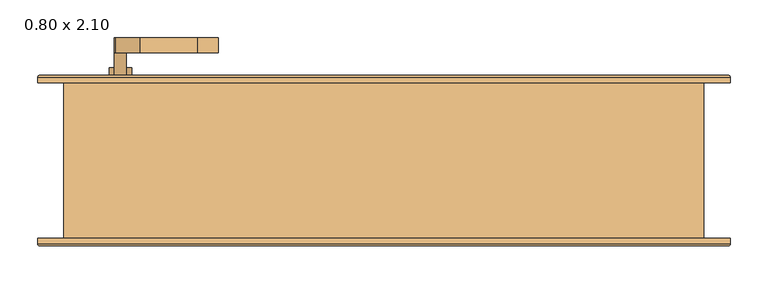
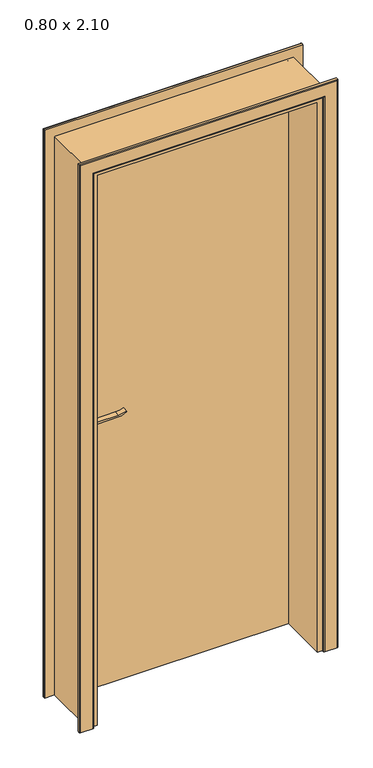
"""IFC4 building model written with IfcOpenShell, lengths in millimetres: door geometry, .CC_ND 300_PORTA SIMPLES DE ABRIR_COM EXTENSÃO : 0.80 x 2.10."""

import ifcopenshell
import ifcopenshell.guid

model = None  # the IFC model being written
_history = None  # IfcOwnerHistory: only IFC2X3 demands one
_inside = {}  # id of a spatial element -> (the spatial element, [elements in it])
_under = {}  # id of a project, library or spatial element -> (it, [spatial elements below it])
_declared = {}  # id of a project -> (the project, [libraries it declares])
_typed = {}  # id of a type object -> (the type object, [elements of that type])
_made_of = {}  # id of a material, layer set ... -> (it, [elements and type objects made of it])


def new_model(schema):
    """Start an empty IFC model of exactly this schema.

    Asked for "IFC4X3", IfcOpenShell would pick the latest addendum, in which some entities
    have other attributes; the version numbers below select the first issue.
    IFC2X3 requires an IfcOwnerHistory on every rooted entity: one is made here for all.
    """
    global model, _history
    if schema == "IFC4X3":
        model = ifcopenshell.file(schema_version=(4, 3, 0, 0))
    else:
        model = ifcopenshell.file(schema=schema)
    _inside.clear()
    _under.clear()
    _declared.clear()
    _typed.clear()
    _made_of.clear()
    _history = None
    if model.schema == "IFC2X3":
        org = make("IfcOrganization", Name="unknown")
        user = make(
            "IfcPersonAndOrganization",
            ThePerson=make("IfcPerson", FamilyName="unknown"),
            TheOrganization=org,
        )
        app = make(
            "IfcApplication",
            ApplicationDeveloper=org,
            Version="unknown",
            ApplicationFullName="unknown",
            ApplicationIdentifier="unknown",
        )
        _history = make(
            "IfcOwnerHistory",
            OwningUser=user,
            OwningApplication=app,
            ChangeAction="ADDED",
            CreationDate=0,
        )
    return model


def make(cls, **values):
    """One entity of the class cls with the attributes given. An attribute that is None is left unset."""
    return model.create_entity(
        cls, **{name: value for name, value in values.items() if value is not None}
    )


def rooted(cls, **values):
    """An entity with a GlobalId (a new one), such as an element, a storey or a relation."""
    return make(cls, GlobalId=ifcopenshell.guid.new(), OwnerHistory=_history, **values)


def si_unit(unit_type, name, prefix=None):
    """IfcSIUnit, for example si_unit("LENGTHUNIT", "METRE", prefix="MILLI")."""
    return make("IfcSIUnit", UnitType=unit_type, Prefix=prefix, Name=name)


def assignment(units):
    """IfcUnitAssignment: the units of a project."""
    return None if units is None else make("IfcUnitAssignment", Units=units)


def point(xyz):
    """IfcCartesianPoint."""
    return None if xyz is None else make("IfcCartesianPoint", Coordinates=xyz)


def direction(xyz):
    """IfcDirection."""
    return None if xyz is None else make("IfcDirection", DirectionRatios=xyz)


def frame(location, z_axis=None, x_axis=None):
    """IfcAxis2Placement3D, a coordinate frame: its origin and axes. An axis left out is left unset."""
    return make(
        "IfcAxis2Placement3D",
        Location=point(location),
        Axis=direction(z_axis),
        RefDirection=direction(x_axis),
    )


def frame_2d(location, x_axis=None):
    """IfcAxis2Placement2D, a coordinate frame in the plane: its origin and x axis."""
    return make(
        "IfcAxis2Placement2D", Location=point(location), RefDirection=direction(x_axis)
    )


def origin():
    """The frame at (0, 0, 0) with its axes left unset."""
    return frame((0.0, 0.0, 0.0))


def origin_with_axes():
    """The frame at (0, 0, 0) with the z axis (0, 0, 1) and the x axis (1, 0, 0) written out."""
    return frame((0.0, 0.0, 0.0), z_axis=(0.0, 0.0, 1.0), x_axis=(1.0, 0.0, 0.0))


def place(relative_to, where):
    """IfcLocalPlacement: puts the frame where relative to a parent placement (None: the world)."""
    return make(
        "IfcLocalPlacement", PlacementRelTo=relative_to, RelativePlacement=where
    )


def context(
    kind, dimensions, precision=None, world=None, true_north=None, identifier=None
):
    """IfcGeometricRepresentationContext, for example the 3D "Model" context."""
    return make(
        "IfcGeometricRepresentationContext",
        ContextIdentifier=identifier,
        ContextType=kind,
        CoordinateSpaceDimension=dimensions,
        Precision=precision,
        WorldCoordinateSystem=world,
        TrueNorth=true_north,
    )


def project(units=None, contexts=None):
    """IfcProject with its units and contexts."""
    return rooted(
        "IfcProject",
        Name="project",
        RepresentationContexts=contexts,
        UnitsInContext=assignment(units),
    )


def spatial(cls, under=None, at=None, **own):
    """A site, building, storey or space (cls), placed at a placement, below another one or the project."""
    s = rooted(cls, ObjectPlacement=at, **own)
    if under is not None:
        _under.setdefault(under.id(), (under, []))[1].append(s)
    return s


def polyline(points):
    """IfcPolyline through the points."""
    return make("IfcPolyline", Points=[point(p) for p in points])


def circle_curve(where, radius):
    """IfcCircle in the frame where."""
    return make("IfcCircle", Position=where, Radius=radius)


def ellipse_curve(where, semi_axis1, semi_axis2):
    """IfcEllipse in the frame where."""
    return make(
        "IfcEllipse", Position=where, SemiAxis1=semi_axis1, SemiAxis2=semi_axis2
    )


def trimmed(basis, trim1, trim2, sense, master):
    """IfcTrimmedCurve: the piece of a basis curve between two trims."""
    return make(
        "IfcTrimmedCurve",
        BasisCurve=basis,
        Trim1=trim1,
        Trim2=trim2,
        SenseAgreement=sense,
        MasterRepresentation=master,
    )


def segment(curve, same_sense, transition):
    """IfcCompositeCurveSegment."""
    return make(
        "IfcCompositeCurveSegment",
        Transition=transition,
        SameSense=same_sense,
        ParentCurve=curve,
    )


def composite_curve(segments, self_intersect=None):
    """IfcCompositeCurve: segments joined end to end."""
    return make("IfcCompositeCurve", Segments=segments, SelfIntersect=self_intersect)


def outline(outer, holes=None, kind="AREA"):
    """IfcArbitraryClosedProfileDef: a profile drawn as a closed curve; with holes, ...WithVoids."""
    if holes is None:
        return make("IfcArbitraryClosedProfileDef", ProfileType=kind, OuterCurve=outer)
    return make(
        "IfcArbitraryProfileDefWithVoids",
        ProfileType=kind,
        OuterCurve=outer,
        InnerCurves=holes,
    )


def extrude(swept, where, along, depth):
    """IfcExtrudedAreaSolid: the profile swept, set in the frame where, extruded along a direction by depth."""
    return make(
        "IfcExtrudedAreaSolid",
        SweptArea=swept,
        Position=where,
        ExtrudedDirection=direction(along),
        Depth=depth,
    )


def faces_of(points, faces, orient=None, outer=None):
    """IfcFace entities. A face is a list of loops; a loop is a list of indices into points, from 0.

    orient and outer hold one flag for each loop. By default every Orientation is true, the
    first loop of a face is its IfcFaceOuterBound and the others are IfcFaceBound.
    """
    made = []
    for i, loops in enumerate(faces):
        bounds = []
        for j, loop in enumerate(loops):
            is_outer = j == 0 if outer is None else outer[i][j]
            bounds.append(
                make(
                    "IfcFaceOuterBound" if is_outer else "IfcFaceBound",
                    Bound=make("IfcPolyLoop", Polygon=[points[k] for k in loop]),
                    Orientation=True if orient is None else orient[i][j],
                )
            )
        made.append(make("IfcFace", Bounds=bounds))
    return made


def faceted_brep(points, faces, orient=None, outer=None, voids=None):
    """IfcFacetedBrep: a solid bounded by flat faces; with voids (closed shells), ...WithVoids."""
    shared = [point(p) for p in points]
    hull = make("IfcClosedShell", CfsFaces=faces_of(shared, faces, orient, outer))
    if voids is None:
        return make("IfcFacetedBrep", Outer=hull)
    return make(
        "IfcFacetedBrepWithVoids",
        Outer=hull,
        Voids=[
            make(cls, CfsFaces=faces_of(shared, fs, o, b)) for cls, fs, o, b in voids
        ],
    )


def shape(context_of_items, identifier, shape_type, items):
    """IfcShapeRepresentation: the items that make up one representation, for example the "Body"."""
    return make(
        "IfcShapeRepresentation",
        ContextOfItems=context_of_items,
        RepresentationIdentifier=identifier,
        RepresentationType=shape_type,
        Items=items,
    )


def source(mapping_origin, context_of_items, identifier, shape_type, items):
    """IfcRepresentationMap: a shape defined once, which mapped items show again and again."""
    return make(
        "IfcRepresentationMap",
        MappingOrigin=mapping_origin,
        MappedRepresentation=shape(context_of_items, identifier, shape_type, items),
    )


def transform(
    local_origin,
    x_axis=None,
    y_axis=None,
    z_axis=None,
    scale=None,
    scale2=None,
    scale3=None,
    uniform=True,
):
    """IfcCartesianTransformationOperator3D, or its non-uniform kind. x_axis, y_axis, z_axis: its Axis1, 2, 3."""
    if uniform:
        return make(
            "IfcCartesianTransformationOperator3D",
            Axis1=direction(x_axis),
            Axis2=direction(y_axis),
            LocalOrigin=point(local_origin),
            Scale=scale,
            Axis3=direction(z_axis),
        )
    return make(
        "IfcCartesianTransformationOperator3DnonUniform",
        Axis1=direction(x_axis),
        Axis2=direction(y_axis),
        LocalOrigin=point(local_origin),
        Scale=scale,
        Axis3=direction(z_axis),
        Scale2=scale2,
        Scale3=scale3,
    )


def mapped(mapping_source, mapping_target):
    """IfcMappedItem: shows the shape of a source again, moved by a transform."""
    return make(
        "IfcMappedItem", MappingSource=mapping_source, MappingTarget=mapping_target
    )


def made_of(thing, what):
    """Note that an element or type object is made of a material, layer set ...; save() writes the relation."""
    if what is not None:
        _made_of.setdefault(what.id(), (what, []))[1].append(thing)
    return thing


def element(
    cls,
    number,
    at=None,
    inside=None,
    cuts=None,
    type_object=None,
    material=None,
    context=None,
    identifier="Body",
    shape_type=None,
    held_by="IfcProductDefinitionShape",
    body=None,
    shapes=None,
    **own,
):
    """One element of the class cls, such as IfcWall. Its Tag is "e" and its number.

    at: its placement. inside: the storey or other place that contains it. cuts: it is an
    opening in that element (IfcRelVoidsElement). A single representation is given by context,
    identifier, shape_type and body (its items); several are given by shapes. held_by: the class
    of the entity that holds the representations. save() writes the other relations.
    """
    e = rooted(cls, Tag="e%d" % number, ObjectPlacement=at, **own)
    if body is not None:
        shapes = [shape(context, identifier, shape_type, body)]
    if shapes is not None:
        e.Representation = make(held_by, Representations=shapes)
    if inside is not None:
        _inside.setdefault(inside.id(), (inside, []))[1].append(e)
    if cuts is not None:
        rooted(
            "IfcRelVoidsElement", RelatingBuildingElement=cuts, RelatedOpeningElement=e
        )
    if type_object is not None:
        _typed.setdefault(type_object.id(), (type_object, []))[1].append(e)
    return made_of(e, material)


def aggregate(whole, parts):
    """IfcRelAggregates: a whole, such as a stair, and the parts it consists of."""
    return rooted("IfcRelAggregates", RelatingObject=whole, RelatedObjects=parts)


def save(model, path):
    """Write the relations noted so far, then the file.

    IfcRelAggregates (storeys below a building ...), IfcRelContainedInSpatialStructure (elements
    in a storey), IfcRelDefinesByType, IfcRelAssociatesMaterial and IfcRelDeclares: one each for
    every whole, place, type object, material and project.
    """
    for whole, parts in _under.values():
        aggregate(whole, parts)
    for where, things in _inside.values():
        rooted(
            "IfcRelContainedInSpatialStructure",
            RelatedElements=things,
            RelatingStructure=where,
        )
    for kind, things in _typed.values():
        rooted("IfcRelDefinesByType", RelatedObjects=things, RelatingType=kind)
    for what, things in _made_of.values():
        rooted("IfcRelAssociatesMaterial", RelatedObjects=things, RelatingMaterial=what)
    for by, libraries in _declared.values():
        rooted("IfcRelDeclares", RelatingContext=by, RelatedDefinitions=libraries)
    model.write(path)


def plane_surface(at):
    """IfcPlane: the flat surface through the origin of the frame at, square to its z axis."""
    return make("IfcPlane", Position=at)


def cylinder_surface(at, radius):
    """IfcCylindricalSurface: all points at the distance radius from the z axis of the frame at."""
    return make("IfcCylindricalSurface", Position=at, Radius=radius)


def advanced_brep(points, edges, surfaces, faces):
    """IfcAdvancedBrep: a solid bounded by faces that lie on surfaces and meet in shared edges.

    An edge is (start, end): straight between two places in points (the first is 0);
    or (start, end, curve); or (start, end, curve, False) where it runs against its curve.
    A face is (place in surfaces, loops), or (place, loops, False) where it looks against
    its surface's normal. A loop lists edges by number (the first is 1), with a minus sign
    where the edge is run from its end to its start. The first loop is the outer one.
    """
    corners = [point(p) for p in points]
    vertices = [make("IfcVertexPoint", VertexGeometry=c) for c in corners]
    made = []
    for start, end, *more in edges:
        made.append(
            make(
                "IfcEdgeCurve",
                EdgeStart=vertices[start],
                EdgeEnd=vertices[end],
                EdgeGeometry=more[0] if more else make("IfcPolyline", Points=[corners[start], corners[end]]),
                SameSense=more[1] if len(more) > 1 else True,
            )
        )
    hull = []
    for where, loops, *sense in faces:
        bounds = []
        for j, loop in enumerate(loops):
            ring = [make("IfcOrientedEdge", EdgeElement=made[abs(k) - 1], Orientation=k > 0) for k in loop]
            bounds.append(
                make(
                    "IfcFaceOuterBound" if j == 0 else "IfcFaceBound",
                    Bound=make("IfcEdgeLoop", EdgeList=ring),
                    Orientation=True,
                )
            )
        hull.append(make("IfcAdvancedFace", Bounds=bounds, FaceSurface=surfaces[where], SameSense=sense[0] if sense else True))
    return make("IfcAdvancedBrep", Outer=make("IfcClosedShell", CfsFaces=hull))


def door_0_80_x_2_10_4cab1925(model_context):
    return source(origin(), model_context, "Body", "SolidModel", [
        extrude(outline(composite_curve([segment(trimmed(circle_curve(frame_2d((964.5, -350.0)), 15.0), [point((964.5, -335.0))], [point((964.5, -365.0))], False, "CARTESIAN"), True, "CONTINUOUS"), segment(trimmed(circle_curve(frame_2d((964.5, -350.0)), 15.0), [point((964.5, -365.0))], [point((964.5, -335.0))], False, "CARTESIAN"), True, "CONTINUOUS")], self_intersect=False)), frame((0.0, 110.7, 0.0), z_axis=(0.0, 1.0, 0.0), x_axis=(0.0, 0.0, 1.0)), (0.0, 0.0, 1.0), 10.0),
        extrude(outline(composite_curve([segment(trimmed(circle_curve(frame_2d((964.5, -350.0)), 15.0), [point((964.5, -335.0))], [point((964.5, -365.0))], False, "CARTESIAN"), True, "CONTINUOUS"), segment(trimmed(circle_curve(frame_2d((964.5, -350.0)), 15.0), [point((964.5, -365.0))], [point((964.5, -335.0))], False, "CARTESIAN"), True, "CONTINUOUS")], self_intersect=False)), frame((0.0, 50.7, 0.0), z_axis=(0.0, 1.0, 0.0), x_axis=(0.0, 0.0, 1.0)), (0.0, 0.0, 1.0), 10.0),
        extrude(outline(composite_curve([segment(trimmed(circle_curve(frame_2d((1024.5, -350.0)), 8.0), [point((1029.1523287, -356.5081363))], [point((1024.5, -342.0))], False, "CARTESIAN"), True, "CONTINUOUS"), segment(trimmed(circle_curve(frame_2d((1019.3738613, -324.6138099)), 18.1261387), [point((1024.5, -342.0))], [point((1037.5, -324.6138099))], True, "CARTESIAN"), True, "CONTINUOUS"), segment(polyline([(1037.5, -324.6138099), (1037.5, -248.3564091)]), True, "CONTINUOUS"), segment(trimmed(circle_curve(frame_2d((1096.7709207, -251.9396612)), 59.3791355), [point((1037.5, -248.3564091))], [point((1046.7135558, -220.0))], False, "CARTESIAN"), True, "CONTINUOUS"), segment(polyline([(1046.7135558, -220.0), (1049.5, -220.0)]), True, "CONTINUOUS"), segment(trimmed(circle_curve(frame_2d((1127.7850638, -248.4227909)), 83.2850902), [point((1049.5, -220.0))], [point((1044.5, -248.3564091))], True, "CARTESIAN"), True, "CONTINUOUS"), segment(polyline([(1044.5, -248.3564091), (1044.5, -324.6325667)]), True, "CONTINUOUS"), segment(trimmed(circle_curve(frame_2d((1007.2555521, -326.3324871)), 37.2832219), [point((1044.5, -324.6325667))], [point((1029.1523287, -356.5081363))], False, "CARTESIAN"), True, "CONTINUOUS")], self_intersect=False)), frame((0.0, 140.7, 0.0), z_axis=(0.0, 1.0, 0.0), x_axis=(0.0, 0.0, 1.0)), (0.0, 0.0, 1.0), 20.0),
        extrude(outline(composite_curve([segment(trimmed(circle_curve(frame_2d((1019.3738682, -324.6138122)), 18.1261318), [point((1024.4999903, -342.0))], [point((1037.5, -324.6138122))], True, "CARTESIAN"), True, "CONTINUOUS"), segment(polyline([(1037.5, -324.6138122), (1037.5, -248.3564091)]), True, "CONTINUOUS"), segment(trimmed(circle_curve(frame_2d((1096.7709207, -251.9396612)), 59.3791355), [point((1037.5, -248.3564091))], [point((1046.7135558, -220.0))], False, "CARTESIAN"), True, "CONTINUOUS"), segment(polyline([(1046.7135558, -220.0), (1049.5, -220.0)]), True, "CONTINUOUS"), segment(trimmed(circle_curve(frame_2d((1127.7850638, -248.4227909)), 83.2850902), [point((1049.5, -220.0))], [point((1044.5, -248.3564091))], True, "CARTESIAN"), True, "CONTINUOUS"), segment(polyline([(1044.5, -248.3564091), (1044.5, -324.6325667)]), True, "CONTINUOUS"), segment(trimmed(circle_curve(frame_2d((1007.2555521, -326.3324871)), 37.2832219), [point((1044.5, -324.6325667))], [point((1029.1523287, -356.5081363))], False, "CARTESIAN"), True, "CONTINUOUS"), segment(trimmed(circle_curve(frame_2d((1024.5, -350.0)), 8.0), [point((1029.1523287, -356.5081363))], [point((1024.4999903, -342.0))], False, "CARTESIAN"), True, "CONTINUOUS")], self_intersect=False)), frame((0.0, 10.7, 0.0), z_axis=(0.0, 1.0, 0.0), x_axis=(0.0, 0.0, 1.0)), (0.0, 0.0, 1.0), 20.0),
        extrude(outline(composite_curve([segment(trimmed(circle_curve(frame_2d((1024.5, -350.0)), 8.0), [point((1024.5, -342.0))], [point((1024.5, -358.0))], False, "CARTESIAN"), True, "CONTINUOUS"), segment(trimmed(circle_curve(frame_2d((1024.5, -350.0)), 8.0), [point((1024.5, -358.0))], [point((1024.5, -342.0))], False, "CARTESIAN"), True, "CONTINUOUS")], self_intersect=False)), frame((0.0, 110.7, 0.0), z_axis=(0.0, 1.0, 0.0), x_axis=(0.0, 0.0, 1.0)), (0.0, 0.0, 1.0), 30.0),
        extrude(outline(composite_curve([segment(trimmed(circle_curve(frame_2d((1024.5, -350.0)), 8.0), [point((1024.5, -342.0))], [point((1024.5, -358.0))], False, "CARTESIAN"), True, "CONTINUOUS"), segment(trimmed(circle_curve(frame_2d((1024.5, -350.0)), 8.0), [point((1024.5, -358.0))], [point((1024.5, -342.0))], False, "CARTESIAN"), True, "CONTINUOUS")], self_intersect=False)), frame((0.0, 30.7, 0.0), z_axis=(0.0, 1.0, 0.0), x_axis=(0.0, 0.0, 1.0)), (0.0, 0.0, 1.0), 30.0),
        extrude(outline(composite_curve([segment(trimmed(circle_curve(frame_2d((954.5, -350.0)), 25.0), [point((954.5, -375.0))], [point((954.5, -325.0))], False, "CARTESIAN"), True, "CONTINUOUS"), segment(polyline([(954.5, -325.0), (1024.5, -325.0)]), True, "CONTINUOUS"), segment(trimmed(circle_curve(frame_2d((1024.5, -350.0)), 25.0), [point((1024.5, -325.0))], [point((1024.5, -375.0))], False, "CARTESIAN"), True, "CONTINUOUS"), segment(polyline([(1024.5, -375.0), (954.5, -375.0)]), True, "CONTINUOUS")], self_intersect=False)), frame((0.0, 100.7, 0.0), z_axis=(0.0, 1.0, 0.0), x_axis=(0.0, 0.0, 1.0)), (0.0, 0.0, 1.0), 10.0),
        extrude(outline(composite_curve([segment(trimmed(circle_curve(frame_2d((954.5, -350.0)), 25.0), [point((954.5, -375.0))], [point((954.5, -325.0))], False, "CARTESIAN"), True, "CONTINUOUS"), segment(polyline([(954.5, -325.0), (1024.5, -325.0)]), True, "CONTINUOUS"), segment(trimmed(circle_curve(frame_2d((1024.5, -350.0)), 25.0), [point((1024.5, -325.0))], [point((1024.5, -375.0))], False, "CARTESIAN"), True, "CONTINUOUS"), segment(polyline([(1024.5, -375.0), (954.5, -375.0)]), True, "CONTINUOUS")], self_intersect=False)), frame((0.0, 60.7, 0.0), z_axis=(0.0, 1.0, 0.0), x_axis=(0.0, 0.0, 1.0)), (0.0, 0.0, 1.0), 10.0),
        advanced_brep(
        [(-460.0, 100.7, 0.0), (-460.0, 107.7, 0.0), (-457.0, 110.7, 0.0), (-413.0, 110.7, 0.0), (-410.0, 107.7, 0.0), (-410.0, 100.7, 0.0), (-410.0, 100.7, 2085.0), (410.0, 100.7, 2085.0), (410.0, 100.7, 0.0), (460.0, 100.7, 0.0), (460.0, 100.7, 2135.0), (-460.0, 100.7, 2135.0), (-410.0, 107.7, 2085.0), (-413.0, 110.7, 2088.0), (-457.0, 110.7, 2132.0), (457.0, 110.7, 2132.0), (457.0, 110.7, 0.0), (413.0, 110.7, 0.0), (413.0, 110.7, 2088.0), (-460.0, 107.7, 2135.0), (460.0, 107.7, 0.0), (460.0, 107.7, 2135.0), (410.0, 107.7, 0.0), (410.0, 107.7, 2085.0)],
        [
            (0, 1),
            (1, 2, circle_curve(frame((-457.0, 107.7, 0.0), z_axis=(0.0, 0.0, -1.0), x_axis=(1.0, 0.0, 0.0)), 3.0)),
            (2, 3),
            (3, 4, circle_curve(frame((-413.0, 107.7, 0.0), z_axis=(0.0, 0.0, -1.0), x_axis=(1.0, 0.0, 0.0)), 3.0)),
            (4, 5),
            (5, 0),
            (5, 6),
            (6, 7),
            (7, 8),
            (8, 9),
            (9, 10),
            (10, 11),
            (11, 0),
            (4, 12),
            (12, 6),
            (3, 13),
            (13, 12, ellipse_curve(frame((-413.0, 107.7, 2088.0), z_axis=(-0.7071067811865475, 0.0, -0.7071067811865475), x_axis=(0.7071067811865474, 0.0, -0.7071067811865476)), 4.2426407, 3.0)),
            (2, 14),
            (14, 15),
            (15, 16),
            (16, 17),
            (17, 18),
            (18, 13),
            (1, 19),
            (19, 14, ellipse_curve(frame((-457.0, 107.7, 2132.0), z_axis=(-0.7071067811865475, 0.0, -0.7071067811865475), x_axis=(0.7071067811865474, 0.0, -0.7071067811865476)), 4.2426407, 3.0)),
            (11, 19),
            (9, 20),
            (20, 21),
            (21, 10),
            (8, 22),
            (22, 17, circle_curve(frame((413.0, 107.7, 0.0), z_axis=(0.0, 0.0, -1.0), x_axis=(-1.0, 0.0, 0.0)), 3.0)),
            (16, 20, circle_curve(frame((457.0, 107.7, 0.0), z_axis=(0.0, 0.0, -1.0), x_axis=(-1.0, 0.0, 0.0)), 3.0)),
            (23, 22),
            (7, 23),
            (23, 18, ellipse_curve(frame((413.0, 107.7, 2088.0), z_axis=(0.7071067811865475, 0.0, -0.7071067811865475), x_axis=(0.7071067811865474, 0.0, 0.7071067811865476)), 4.2426407, 3.0)),
            (15, 21, ellipse_curve(frame((457.0, 107.7, 2132.0), z_axis=(0.7071067811865475, 0.0, -0.7071067811865475), x_axis=(0.7071067811865474, 0.0, 0.7071067811865476)), 4.2426407, 3.0)),
            (12, 23),
            (21, 19),
        ],
        [
            plane_surface(frame((-410.0, 100.7, 0.0), z_axis=(0.0, 0.0, -1.0), x_axis=(0.0, -1.0, 0.0))),
            plane_surface(frame((-460.0, 100.7, 0.0), z_axis=(0.0, -1.0, 0.0), x_axis=(0.0, 0.0, 1.0))),
            plane_surface(frame((-410.0, 100.7, 0.0), z_axis=(1.0, 0.0, 0.0), x_axis=(0.0, 0.0, 1.0))),
            cylinder_surface(frame((-413.0, 107.7, 0.0), z_axis=(0.0, 0.0, -1.0), x_axis=(1.0, 0.0, 0.0)), 3.0),
            plane_surface(frame((-413.0, 110.7, 0.0), z_axis=(0.0, 1.0, 0.0), x_axis=(0.0, 0.0, 1.0))),
            cylinder_surface(frame((-457.0, 107.7, 0.0), z_axis=(0.0, 0.0, -1.0), x_axis=(1.0, 0.0, 0.0)), 3.0),
            plane_surface(frame((-460.0, 107.7, 0.0), z_axis=(-1.0, 0.0, 0.0), x_axis=(0.0, 0.0, 1.0))),
            plane_surface(frame((460.0, 107.7, 2135.0), z_axis=(1.0, 0.0, 0.0), x_axis=(0.0, 0.0, -1.0))),
            plane_surface(frame((410.0, 100.7, 0.0), z_axis=(0.0, 0.0, -1.0), x_axis=(0.0, -1.0, 0.0))),
            plane_surface(frame((410.0, 100.7, 2085.0), z_axis=(-1.0, 0.0, 0.0), x_axis=(0.0, 0.0, -1.0))),
            cylinder_surface(frame((413.0, 107.7, 2085.0), z_axis=(0.0, 0.0, 1.0), x_axis=(-1.0, 0.0, 0.0)), 3.0),
            cylinder_surface(frame((457.0, 107.7, 2085.0), z_axis=(0.0, 0.0, 1.0), x_axis=(-1.0, 0.0, 0.0)), 3.0),
            plane_surface(frame((-410.0, 100.7, 2085.0), z_axis=(0.0, 0.0, -1.0), x_axis=(1.0, 0.0, 0.0))),
            plane_surface(frame((-460.0, 107.7, 2135.0), z_axis=(0.0, 0.0, 1.0), x_axis=(1.0, 0.0, 0.0))),
            cylinder_surface(frame((-410.0, 107.7, 2088.0), z_axis=(-1.0, 0.0, 0.0), x_axis=(0.0, 0.0, -1.0)), 3.0),
            cylinder_surface(frame((-410.0, 107.7, 2132.0), z_axis=(-1.0, 0.0, 0.0), x_axis=(0.0, 0.0, -1.0)), 3.0),
        ],
        [
            (0, [[1, 2, 3, 4, 5, 6]]),
            (1, [[7, 8, 9, 10, 11, 12, 13, -6]]),
            (2, [[14, 15, -7, -5]]),
            (3, [[16, 17, -14, -4]]),
            (4, [[18, 19, 20, 21, 22, 23, -16, -3]]),
            (5, [[24, 25, -18, -2]]),
            (6, [[-13, 26, -24, -1]]),
            (7, [[-11, 27, 28, 29]]),
            (8, [[-10, 30, 31, -21, 32, -27]]),
            (9, [[33, -30, -9, 34]]),
            (10, [[-22, -31, -33, 35]]),
            (11, [[-28, -32, -20, 36]]),
            (12, [[37, -34, -8, -15]]),
            (13, [[-12, -29, 38, -26]]),
            (14, [[-23, -35, -37, -17]]),
            (15, [[-38, -36, -19, -25]]),
        ],
    ),
        advanced_brep(
        [(460.0, -106.0, 0.0), (460.0, -113.0342217, 0.0), (457.0342217, -116.0, 0.0), (412.9842717, -116.0, 0.0), (410.0, -113.0157283, 0.0), (410.0, -106.0, 0.0), (410.0, -106.0, 2085.0), (-410.0, -106.0, 2085.0), (-410.0, -106.0, 0.0), (-460.0, -106.0, 0.0), (-460.0, -106.0, 2135.0), (460.0, -106.0, 2135.0), (410.0, -113.0157283, 2085.0), (412.9842717, -116.0, 2087.9842717), (457.0342217, -116.0, 2132.0342217), (-457.0342217, -116.0, 2132.0342217), (-457.0342217, -116.0, 0.0), (-412.9842717, -116.0, 0.0), (-412.9842717, -116.0, 2087.9842717), (460.0, -113.0342217, 2135.0), (-460.0, -113.0342217, 0.0), (-460.0, -113.0342217, 2135.0), (-410.0, -113.0157283, 0.0), (-410.0, -113.0157283, 2085.0)],
        [
            (0, 1),
            (1, 2, circle_curve(frame((457.0342217, -113.0342217, 0.0), z_axis=(0.0, 0.0, -1.0), x_axis=(1.0, 0.0, 0.0)), 2.9657783)),
            (2, 3),
            (3, 4, circle_curve(frame((412.9842717, -113.0157283, 0.0), z_axis=(0.0, 0.0, -1.0), x_axis=(1.0, 0.0, 0.0)), 2.9842717)),
            (4, 5),
            (5, 0),
            (5, 6),
            (6, 7),
            (7, 8),
            (8, 9),
            (9, 10),
            (10, 11),
            (11, 0),
            (4, 12),
            (12, 6),
            (3, 13),
            (13, 12, ellipse_curve(frame((412.9842717, -113.0157283, 2087.9842717), z_axis=(0.7071067811865475, 0.0, -0.7071067811865475), x_axis=(-0.7071067811865474, 0.0, -0.7071067811865476)), 4.2203975, 2.9842717)),
            (2, 14),
            (14, 15),
            (15, 16),
            (16, 17),
            (17, 18),
            (18, 13),
            (1, 19),
            (19, 14, ellipse_curve(frame((457.0342217, -113.0342217, 2132.0342217), z_axis=(0.7071067811865475, 0.0, -0.7071067811865475), x_axis=(-0.7071067811865474, 0.0, -0.7071067811865476)), 4.1942438, 2.9657783)),
            (11, 19),
            (9, 20),
            (20, 21),
            (21, 10),
            (8, 22),
            (22, 17, circle_curve(frame((-412.9842717, -113.0157283, 0.0), z_axis=(0.0, 0.0, -1.0), x_axis=(-1.0, 0.0, 0.0)), 2.9842717)),
            (16, 20, circle_curve(frame((-457.0342217, -113.0342217, 0.0), z_axis=(0.0, 0.0, -1.0), x_axis=(-1.0, 0.0, 0.0)), 2.9657783)),
            (23, 22),
            (7, 23),
            (23, 18, ellipse_curve(frame((-412.9842717, -113.0157283, 2087.9842717), z_axis=(-0.7071067811865475, 0.0, -0.7071067811865475), x_axis=(-0.7071067811865474, 0.0, 0.7071067811865476)), 4.2203975, 2.9842717)),
            (15, 21, ellipse_curve(frame((-457.0342217, -113.0342217, 2132.0342217), z_axis=(-0.7071067811865475, 0.0, -0.7071067811865475), x_axis=(-0.7071067811865474, 0.0, 0.7071067811865476)), 4.1942438, 2.9657783)),
            (12, 23),
            (21, 19),
        ],
        [
            plane_surface(frame((410.0, -106.0, 0.0), z_axis=(0.0, 0.0, -1.0), x_axis=(0.0, -1.0, 0.0))),
            plane_surface(frame((460.0, -106.0, 0.0), z_axis=(0.0, 1.0, 0.0), x_axis=(0.0, 0.0, 1.0))),
            plane_surface(frame((410.0, -106.0, 0.0), z_axis=(-1.0, 0.0, 0.0), x_axis=(0.0, 0.0, 1.0))),
            cylinder_surface(frame((412.9842717, -113.0157283, 0.0), z_axis=(0.0, 0.0, -1.0), x_axis=(1.0, 0.0, 0.0)), 2.9842717),
            plane_surface(frame((412.9842717, -116.0, 0.0), z_axis=(0.0, -1.0, 0.0), x_axis=(0.0, 0.0, 1.0))),
            cylinder_surface(frame((457.0342217, -113.0342217, 0.0), z_axis=(0.0, 0.0, -1.0), x_axis=(1.0, 0.0, 0.0)), 2.9657783),
            plane_surface(frame((460.0, -113.0342217, 0.0), z_axis=(1.0, 0.0, 0.0), x_axis=(0.0, 0.0, 1.0))),
            plane_surface(frame((-460.0, -113.0342217, 2135.0), z_axis=(-1.0, 0.0, 0.0), x_axis=(0.0, 0.0, -1.0))),
            plane_surface(frame((-410.0, -106.0, 0.0), z_axis=(0.0, 0.0, -1.0), x_axis=(0.0, -1.0, 0.0))),
            plane_surface(frame((-410.0, -106.0, 2085.0), z_axis=(1.0, 0.0, 0.0), x_axis=(0.0, 0.0, -1.0))),
            cylinder_surface(frame((-412.9842717, -113.0157283, 2085.0), z_axis=(0.0, 0.0, 1.0), x_axis=(-1.0, 0.0, 0.0)), 2.9842717),
            cylinder_surface(frame((-457.0342217, -113.0342217, 2085.0), z_axis=(0.0, 0.0, 1.0), x_axis=(-1.0, 0.0, 0.0)), 2.9657783),
            plane_surface(frame((410.0, -106.0, 2085.0), z_axis=(0.0, 0.0, -1.0), x_axis=(-1.0, 0.0, 0.0))),
            plane_surface(frame((460.0, -113.0342217, 2135.0), z_axis=(0.0, 0.0, 1.0), x_axis=(-1.0, 0.0, 0.0))),
            cylinder_surface(frame((410.0, -113.0157283, 2087.9842717), z_axis=(1.0, 0.0, 0.0), x_axis=(0.0, 0.0, 1.0)), 2.9842717),
            cylinder_surface(frame((410.0, -113.0342217, 2132.0342217), z_axis=(1.0, 0.0, 0.0), x_axis=(0.0, 0.0, 1.0)), 2.9657783),
        ],
        [
            (0, [[1, 2, 3, 4, 5, 6]]),
            (1, [[7, 8, 9, 10, 11, 12, 13, -6]]),
            (2, [[14, 15, -7, -5]]),
            (3, [[16, 17, -14, -4]]),
            (4, [[18, 19, 20, 21, 22, 23, -16, -3]]),
            (5, [[24, 25, -18, -2]]),
            (6, [[-13, 26, -24, -1]]),
            (7, [[-11, 27, 28, 29]]),
            (8, [[-10, 30, 31, -21, 32, -27]]),
            (9, [[33, -30, -9, 34]]),
            (10, [[-22, -31, -33, 35]]),
            (11, [[-28, -32, -20, 36]]),
            (12, [[37, -34, -8, -15]]),
            (13, [[-12, -29, 38, -26]]),
            (14, [[-23, -35, -37, -17]]),
            (15, [[-38, -36, -19, -25]]),
        ],
    ),
        faceted_brep([(392.0, -106.0, 0.0), (392.0, 70.7, 0.0), (400.0, 70.7, 0.0), (400.0, 100.7, 0.0), (425.0, 100.7, 0.0), (425.0, -106.0, 0.0), (425.0, -106.0, 2100.0), (-425.0, -106.0, 2100.0), (-425.0, -106.0, 0.0), (-392.0, -106.0, 0.0), (-392.0, -106.0, 2067.0), (392.0, -106.0, 2067.0), (425.0, 100.7, 2100.0), (400.0, 100.7, 2075.0), (-400.0, 100.7, 2075.0), (-400.0, 100.7, 0.0), (-425.0, 100.7, 0.0), (-425.0, 100.7, 2100.0), (400.0, 70.7, 2075.0), (392.0, 70.7, 2067.0), (-392.0, 70.7, 2067.0), (-392.0, 70.7, 0.0), (-400.0, 70.7, 0.0), (-400.0, 70.7, 2075.0)], [[[0, 1, 2, 3, 4, 5]], [[5, 6, 7, 8, 9, 10, 11, 0]], [[4, 12, 6, 5]], [[3, 13, 14, 15, 16, 17, 12, 4]], [[2, 18, 13, 3]], [[1, 19, 20, 21, 22, 23, 18, 2]], [[0, 11, 19, 1]], [[10, 9, 21, 20]], [[9, 8, 16, 15, 22, 21]], [[17, 16, 8, 7]], [[23, 22, 15, 14]], [[12, 17, 7, 6]], [[18, 23, 14, 13]], [[11, 10, 20, 19]]]),
        extrude(outline(polyline([(-400.0, 70.7), (-400.0, 100.7), (400.0, 100.7), (400.0, 70.7), (-400.0, 70.7)])), origin_with_axes(), (0.0, 0.0, 1.0), 2075.0),
    ])


if __name__ == "__main__":
    model = new_model("IFC4")
    model_context = context("Model", 3, world=origin())
    ifc_project = project(units=[si_unit("LENGTHUNIT", "METRE", prefix="MILLI")], contexts=[model_context])
    site = spatial("IfcSite", under=ifc_project)
    building = spatial("IfcBuilding", under=site)
    placement = place(None, origin())
    door_0_80_x_2_10_shape = door_0_80_x_2_10_4cab1925(model_context)
    element("IfcDoor", 1, ObjectType=".CC_ND 300_PORTA SIMPLES DE ABRIR_COM EXTENSÃO : 0.80 x 2.10", at=placement, inside=building, context=model_context, shape_type="MappedRepresentation", body=[
        mapped(door_0_80_x_2_10_shape, transform((0.0, 0.0, 0.0), x_axis=(1.0, 0.0, 0.0), y_axis=(0.0, 1.0, 0.0), z_axis=(0.0, 0.0, 1.0))),
    ])
    save(model, "model.ifc")

# Revit data of these elements
# Type ".CC_ND 300_PORTA SIMPLES DE ABRIR_COM EXTENSÃO : 0.80 x 2.10"
#   Type Mark = "153"
#   Rough Width = 0.85 m
#   Espessura moldura externa = 0.01 m
#   Espessura moldura interna = 0.01 m
#   Largura moldura = 0.05 m
#   Extensão acabamento exterior [instance default] = 0.00 m
#   Extensão acabamento interior [instance default] = 0.00 m
#   Espessura batente = 0.025 m
#   Thickness = 0.03 m
#   Altura batente = 2.085 m
#   Aux Arco [instance default] = 0.80 m
#   Rough Height = 2.125 m
#   Height = 2.10 m
#   Width = 0.80 m
#   Moldura interna [instance default] = yes
#   Moldura externa [instance default] = yes
#   Porta = .MADEIRA COM PINTURA ESMALTE BRANCO ACETINADO
#   Moldura = .MADEIRA COM PINTURA ESMALTE BRANCO ACETINADO
#   Maçaneta = .ALUMÍNIO
#   Batente = .MADEIRA COM PINTURA ESMALTE BRANCO ACETINADO
#   Function = (empty or 0)
#   Wall Closure = (empty or 0)
# Element 1 (IfcDoor, ".CC_ND 300_PORTA SIMPLES DE ABRIR_COM EXTENSÃO : 0.80 x 2.10")
#   Extensão acabamento exterior = 0.031 m
#   Extensão acabamento interior = 0.0257 m
#   Aux Arco = 0.8257 m
#   Materials on its faces: ".MADEIRA COM PINTURA ESMALTE BRANCO ACETINADO", ".ALUMÍNIO"
# Materials
#   ".MADEIRA COM PINTURA ESMALTE BRANCO ACETINADO": class ".CC_MADEIRAS", colour RGB 240 240 240, transparency 0, Description = "Madeira com pintura esmalte branco acetinado.", Cost = 0
#   ".ALUMÍNIO": class "CC_METAIS", colour RGB 244 244 244, transparency 0, Description = "Material alumínio", Cost = 0
